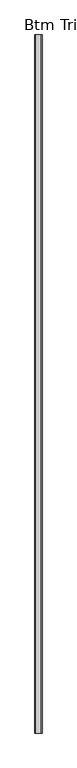
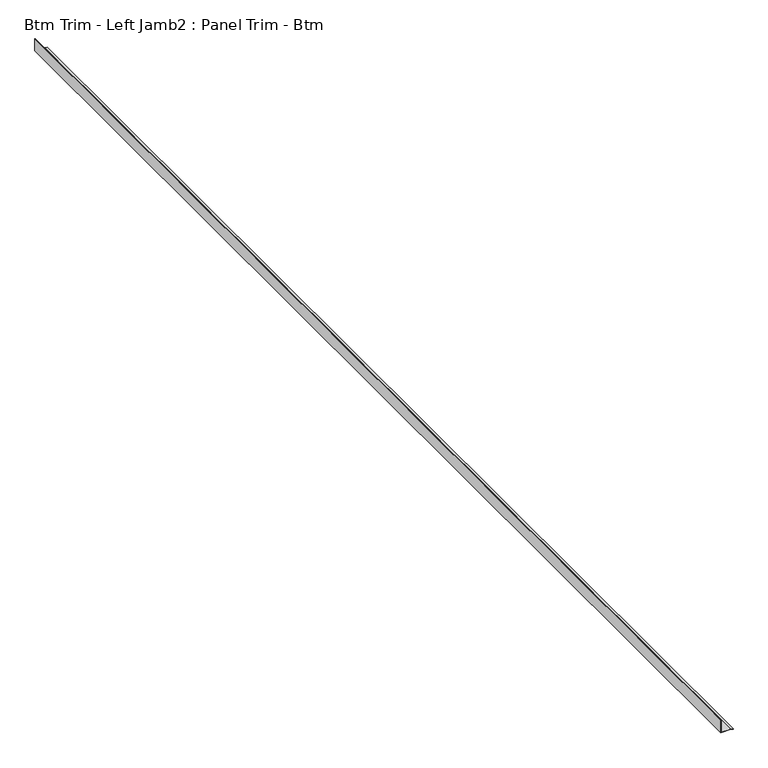
"""IFC4 building model written with IfcOpenShell, lengths in millimetres: proxy geometry, Btm Trim - Left Jamb2 : Panel Trim - Btm."""

from ifc_helpers import new_model, si_unit, frame, origin, place, context, project, spatial, polyline, outline, extrude, source, transform, mapped, element, save


def btm_trim_left_jamb2_panel_trim_btm_415e01f6(model_context):
    return source(origin(), model_context, "Body", "SweptSolid", [
        extrude(outline(polyline([(0.79375, 590391.7729731), (0.79375, 590352.7810739), (51.59375, 590352.7810739), (51.59375, 590351.9936739), (0.0, 590351.9936739), (0.0, 590391.6684739), (-2.4652514, 590400.8689174), (-1.6985478, 590401.074355), (0.79375, 590391.7729731)])), frame((0.0, -536419.2866763, 0.0), z_axis=(0.0, 1.0, 0.0), x_axis=(0.0, 0.0, 1.0)), (0.0, 0.0, 1.0), 4817.5606922),
    ])


if __name__ == "__main__":
    model = new_model("IFC4")
    model_context = context("Model", 3, world=origin())
    ifc_project = project(units=[si_unit("LENGTHUNIT", "METRE", prefix="MILLI")], contexts=[model_context])
    site = spatial("IfcSite", under=ifc_project)
    building = spatial("IfcBuilding", under=site)
    placement = place(None, origin())
    btm_trim_left_jamb2_panel_trim_btm_shape = btm_trim_left_jamb2_panel_trim_btm_415e01f6(model_context)
    element("IfcBuildingElementProxy", 1, Name="Btm Trim - Left Jamb2 : Panel Trim - Btm", ObjectType="Btm Trim - Left Jamb2 : Panel Trim - Btm", at=placement, inside=building, context=model_context, shape_type="MappedRepresentation", body=[
        mapped(btm_trim_left_jamb2_panel_trim_btm_shape, transform((0.0, 0.0, 0.0), x_axis=(1.0, 0.0, 0.0), y_axis=(0.0, 1.0, 0.0), z_axis=(0.0, 0.0, 1.0))),
    ])
    save(model, "model.ifc")

# Revit data of these elements
# Element 1 (IfcBuildingElementProxy, "Btm Trim - Left Jamb2 : Panel Trim - Btm")
#   Materials on its faces: "BASE TRIM BY MTL PANEL MFR."
# Materials
#   "BASE TRIM BY MTL PANEL MFR.": class "Generic", colour RGB 239 242 240, transparency 0, Cost = 0
